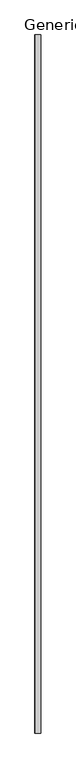
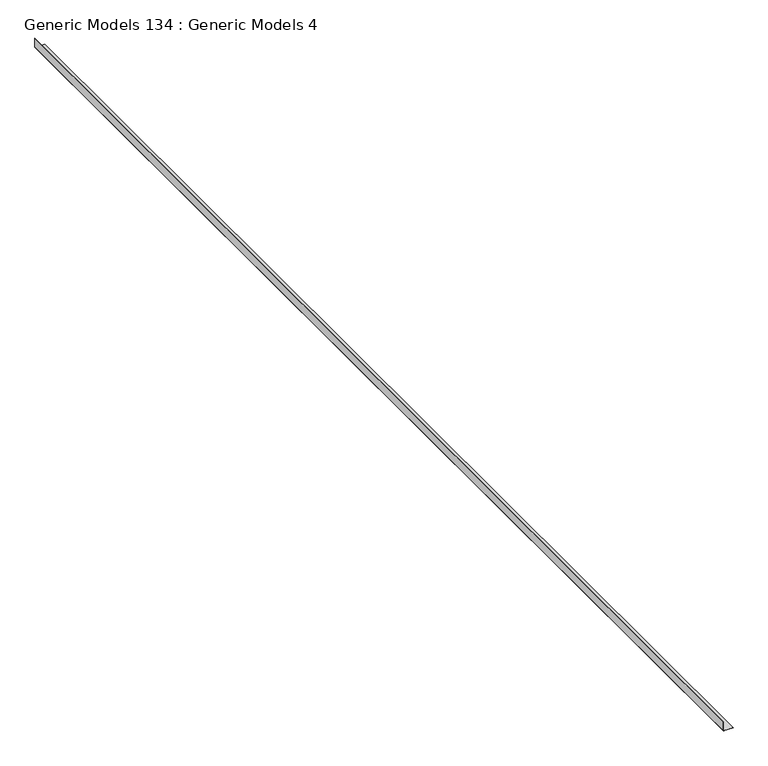
"""IFC4 building model written with IfcOpenShell, lengths in millimetres: proxy geometry, Generic Models 134 : Generic Models 4."""

import ifcopenshell
import ifcopenshell.guid

model = None  # the IFC model being written
_history = None  # IfcOwnerHistory: only IFC2X3 demands one
_inside = {}  # id of a spatial element -> (the spatial element, [elements in it])
_under = {}  # id of a project, library or spatial element -> (it, [spatial elements below it])
_declared = {}  # id of a project -> (the project, [libraries it declares])
_typed = {}  # id of a type object -> (the type object, [elements of that type])
_made_of = {}  # id of a material, layer set ... -> (it, [elements and type objects made of it])


def new_model(schema):
    """Start an empty IFC model of exactly this schema.

    Asked for "IFC4X3", IfcOpenShell would pick the latest addendum, in which some entities
    have other attributes; the version numbers below select the first issue.
    IFC2X3 requires an IfcOwnerHistory on every rooted entity: one is made here for all.
    """
    global model, _history
    if schema == "IFC4X3":
        model = ifcopenshell.file(schema_version=(4, 3, 0, 0))
    else:
        model = ifcopenshell.file(schema=schema)
    _inside.clear()
    _under.clear()
    _declared.clear()
    _typed.clear()
    _made_of.clear()
    _history = None
    if model.schema == "IFC2X3":
        org = make("IfcOrganization", Name="unknown")
        user = make(
            "IfcPersonAndOrganization",
            ThePerson=make("IfcPerson", FamilyName="unknown"),
            TheOrganization=org,
        )
        app = make(
            "IfcApplication",
            ApplicationDeveloper=org,
            Version="unknown",
            ApplicationFullName="unknown",
            ApplicationIdentifier="unknown",
        )
        _history = make(
            "IfcOwnerHistory",
            OwningUser=user,
            OwningApplication=app,
            ChangeAction="ADDED",
            CreationDate=0,
        )
    return model


def make(cls, **values):
    """One entity of the class cls with the attributes given. An attribute that is None is left unset."""
    return model.create_entity(
        cls, **{name: value for name, value in values.items() if value is not None}
    )


def rooted(cls, **values):
    """An entity with a GlobalId (a new one), such as an element, a storey or a relation."""
    return make(cls, GlobalId=ifcopenshell.guid.new(), OwnerHistory=_history, **values)


def si_unit(unit_type, name, prefix=None):
    """IfcSIUnit, for example si_unit("LENGTHUNIT", "METRE", prefix="MILLI")."""
    return make("IfcSIUnit", UnitType=unit_type, Prefix=prefix, Name=name)


def assignment(units):
    """IfcUnitAssignment: the units of a project."""
    return None if units is None else make("IfcUnitAssignment", Units=units)


def point(xyz):
    """IfcCartesianPoint."""
    return None if xyz is None else make("IfcCartesianPoint", Coordinates=xyz)


def direction(xyz):
    """IfcDirection."""
    return None if xyz is None else make("IfcDirection", DirectionRatios=xyz)


def frame(location, z_axis=None, x_axis=None):
    """IfcAxis2Placement3D, a coordinate frame: its origin and axes. An axis left out is left unset."""
    return make(
        "IfcAxis2Placement3D",
        Location=point(location),
        Axis=direction(z_axis),
        RefDirection=direction(x_axis),
    )


def origin():
    """The frame at (0, 0, 0) with its axes left unset."""
    return frame((0.0, 0.0, 0.0))


def place(relative_to, where):
    """IfcLocalPlacement: puts the frame where relative to a parent placement (None: the world)."""
    return make(
        "IfcLocalPlacement", PlacementRelTo=relative_to, RelativePlacement=where
    )


def context(
    kind, dimensions, precision=None, world=None, true_north=None, identifier=None
):
    """IfcGeometricRepresentationContext, for example the 3D "Model" context."""
    return make(
        "IfcGeometricRepresentationContext",
        ContextIdentifier=identifier,
        ContextType=kind,
        CoordinateSpaceDimension=dimensions,
        Precision=precision,
        WorldCoordinateSystem=world,
        TrueNorth=true_north,
    )


def project(units=None, contexts=None):
    """IfcProject with its units and contexts."""
    return rooted(
        "IfcProject",
        Name="project",
        RepresentationContexts=contexts,
        UnitsInContext=assignment(units),
    )


def spatial(cls, under=None, at=None, **own):
    """A site, building, storey or space (cls), placed at a placement, below another one or the project."""
    s = rooted(cls, ObjectPlacement=at, **own)
    if under is not None:
        _under.setdefault(under.id(), (under, []))[1].append(s)
    return s


def polyline(points):
    """IfcPolyline through the points."""
    return make("IfcPolyline", Points=[point(p) for p in points])


def outline(outer, holes=None, kind="AREA"):
    """IfcArbitraryClosedProfileDef: a profile drawn as a closed curve; with holes, ...WithVoids."""
    if holes is None:
        return make("IfcArbitraryClosedProfileDef", ProfileType=kind, OuterCurve=outer)
    return make(
        "IfcArbitraryProfileDefWithVoids",
        ProfileType=kind,
        OuterCurve=outer,
        InnerCurves=holes,
    )


def extrude(swept, where, along, depth):
    """IfcExtrudedAreaSolid: the profile swept, set in the frame where, extruded along a direction by depth."""
    return make(
        "IfcExtrudedAreaSolid",
        SweptArea=swept,
        Position=where,
        ExtrudedDirection=direction(along),
        Depth=depth,
    )


def shape(context_of_items, identifier, shape_type, items):
    """IfcShapeRepresentation: the items that make up one representation, for example the "Body"."""
    return make(
        "IfcShapeRepresentation",
        ContextOfItems=context_of_items,
        RepresentationIdentifier=identifier,
        RepresentationType=shape_type,
        Items=items,
    )


def source(mapping_origin, context_of_items, identifier, shape_type, items):
    """IfcRepresentationMap: a shape defined once, which mapped items show again and again."""
    return make(
        "IfcRepresentationMap",
        MappingOrigin=mapping_origin,
        MappedRepresentation=shape(context_of_items, identifier, shape_type, items),
    )


def transform(
    local_origin,
    x_axis=None,
    y_axis=None,
    z_axis=None,
    scale=None,
    scale2=None,
    scale3=None,
    uniform=True,
):
    """IfcCartesianTransformationOperator3D, or its non-uniform kind. x_axis, y_axis, z_axis: its Axis1, 2, 3."""
    if uniform:
        return make(
            "IfcCartesianTransformationOperator3D",
            Axis1=direction(x_axis),
            Axis2=direction(y_axis),
            LocalOrigin=point(local_origin),
            Scale=scale,
            Axis3=direction(z_axis),
        )
    return make(
        "IfcCartesianTransformationOperator3DnonUniform",
        Axis1=direction(x_axis),
        Axis2=direction(y_axis),
        LocalOrigin=point(local_origin),
        Scale=scale,
        Axis3=direction(z_axis),
        Scale2=scale2,
        Scale3=scale3,
    )


def mapped(mapping_source, mapping_target):
    """IfcMappedItem: shows the shape of a source again, moved by a transform."""
    return make(
        "IfcMappedItem", MappingSource=mapping_source, MappingTarget=mapping_target
    )


def made_of(thing, what):
    """Note that an element or type object is made of a material, layer set ...; save() writes the relation."""
    if what is not None:
        _made_of.setdefault(what.id(), (what, []))[1].append(thing)
    return thing


def element(
    cls,
    number,
    at=None,
    inside=None,
    cuts=None,
    type_object=None,
    material=None,
    context=None,
    identifier="Body",
    shape_type=None,
    held_by="IfcProductDefinitionShape",
    body=None,
    shapes=None,
    **own,
):
    """One element of the class cls, such as IfcWall. Its Tag is "e" and its number.

    at: its placement. inside: the storey or other place that contains it. cuts: it is an
    opening in that element (IfcRelVoidsElement). A single representation is given by context,
    identifier, shape_type and body (its items); several are given by shapes. held_by: the class
    of the entity that holds the representations. save() writes the other relations.
    """
    e = rooted(cls, Tag="e%d" % number, ObjectPlacement=at, **own)
    if body is not None:
        shapes = [shape(context, identifier, shape_type, body)]
    if shapes is not None:
        e.Representation = make(held_by, Representations=shapes)
    if inside is not None:
        _inside.setdefault(inside.id(), (inside, []))[1].append(e)
    if cuts is not None:
        rooted(
            "IfcRelVoidsElement", RelatingBuildingElement=cuts, RelatedOpeningElement=e
        )
    if type_object is not None:
        _typed.setdefault(type_object.id(), (type_object, []))[1].append(e)
    return made_of(e, material)


def aggregate(whole, parts):
    """IfcRelAggregates: a whole, such as a stair, and the parts it consists of."""
    return rooted("IfcRelAggregates", RelatingObject=whole, RelatedObjects=parts)


def save(model, path):
    """Write the relations noted so far, then the file.

    IfcRelAggregates (storeys below a building ...), IfcRelContainedInSpatialStructure (elements
    in a storey), IfcRelDefinesByType, IfcRelAssociatesMaterial and IfcRelDeclares: one each for
    every whole, place, type object, material and project.
    """
    for whole, parts in _under.values():
        aggregate(whole, parts)
    for where, things in _inside.values():
        rooted(
            "IfcRelContainedInSpatialStructure",
            RelatedElements=things,
            RelatingStructure=where,
        )
    for kind, things in _typed.values():
        rooted("IfcRelDefinesByType", RelatedObjects=things, RelatingType=kind)
    for what, things in _made_of.values():
        rooted("IfcRelAssociatesMaterial", RelatedObjects=things, RelatingMaterial=what)
    for by, libraries in _declared.values():
        rooted("IfcRelDeclares", RelatingContext=by, RelatedDefinitions=libraries)
    model.write(path)


def generic_models_134_generic_models_4_f48edd56(model_context):
    return source(origin(), model_context, "Body", "SweptSolid", [
        extrude(outline(polyline([(126908.9761365, 7278.5735688), (127061.3761365, 7278.5735688), (127061.3761365, 7277.7798188), (126908.1987507, 7277.7798188), (126905.0082475, 7430.9239737), (126905.8018253, 7430.9405066), (126908.9761365, 7278.5735688)])), frame((0.0, -6864.9230338, 0.0), z_axis=(0.0, 1.0, 0.0), x_axis=(0.0, 0.0, 1.0)), (0.0, 0.0, 1.0), 18643.6),
    ])


if __name__ == "__main__":
    model = new_model("IFC4")
    model_context = context("Model", 3, world=origin())
    ifc_project = project(units=[si_unit("LENGTHUNIT", "METRE", prefix="MILLI")], contexts=[model_context])
    site = spatial("IfcSite", under=ifc_project)
    building = spatial("IfcBuilding", under=site)
    placement = place(None, origin())
    generic_models_134_generic_models_4_shape = generic_models_134_generic_models_4_f48edd56(model_context)
    element("IfcBuildingElementProxy", 1, Name="Generic Models 134 : Generic Models 4", ObjectType="Generic Models 134 : Generic Models 4", at=placement, inside=building, context=model_context, shape_type="MappedRepresentation", body=[
        mapped(generic_models_134_generic_models_4_shape, transform((0.0, 0.0, 0.0), x_axis=(1.0, 0.0, 0.0), y_axis=(0.0, 1.0, 0.0), z_axis=(0.0, 0.0, 1.0))),
    ])
    save(model, "model.ifc")

# Revit data of these elements
# Element 1 (IfcBuildingElementProxy, "Generic Models 134 : Generic Models 4")
#   Materials on its faces: "_16 GA. COPPER \"L\" FLASHING - (6\" HORZ. LEG - 4\" VERT. LEG)"
# Materials
#   "_16 GA. COPPER \"L\" FLASHING - (6\" HORZ. LEG - 4\" VERT. LEG)": class "Generic", colour RGB 156 184 169, transparency 0, Cost = 0
